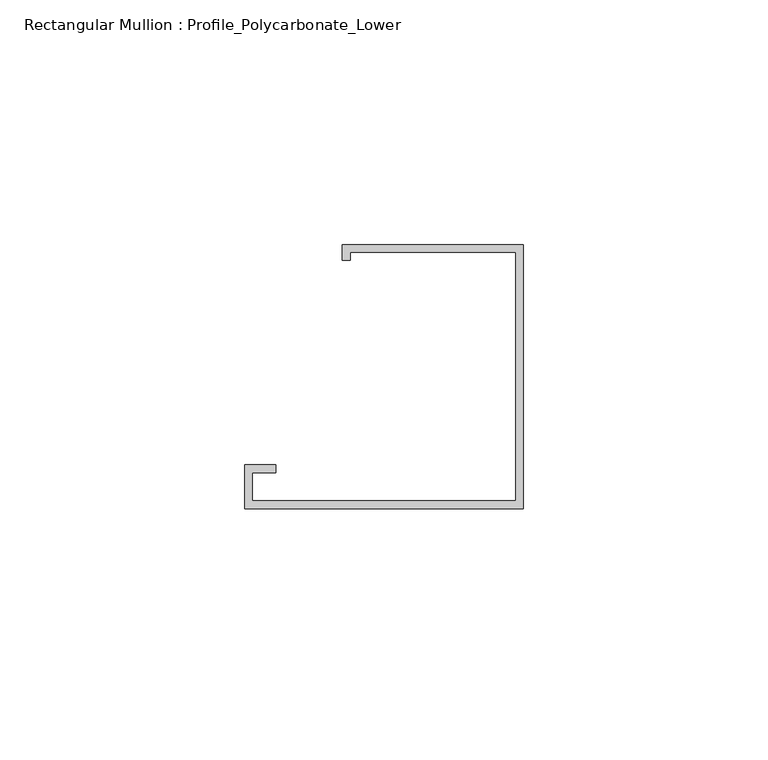
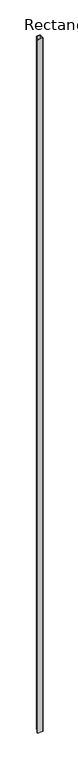
"""IFC4 building model written with IfcOpenShell, lengths in millimetres: member geometry, Rectangular Mullion : Profile_Polycarbonate_Lower."""

from ifc_helpers import new_model, si_unit, frame, origin, place, context, project, spatial, polyline, outline, extrude, source, transform, mapped, element, save


def rectangular_mullion_profile_polycarbonate_lower_ec7f4152(model_context):
    return source(origin(), model_context, "Body", "SweptSolid", [
        extrude(outline(polyline([(0.0, -28.984575), (-56.9976, -28.984575), (-56.9976, -19.992975), (-50.6476, -19.992975), (-50.6476, -21.580475), (-55.4101, -21.580475), (-55.4101, -27.397075), (-1.5875, -27.397075), (-1.5875, 23.428325), (-35.3949, 23.428325), (-35.3949, 21.840825), (-36.9824, 21.840825), (-36.9824, 25.015825), (0.0, 25.015825), (0.0, -28.984575)])), frame((0.0, 0.0, -7626.8283931), z_axis=(0.0, 0.0, 1.0), x_axis=(1.0, 0.0, 0.0)), (0.0, 0.0, 1.0), 7626.8283931),
    ])


if __name__ == "__main__":
    model = new_model("IFC4")
    model_context = context("Model", 3, world=origin())
    ifc_project = project(units=[si_unit("LENGTHUNIT", "METRE", prefix="MILLI")], contexts=[model_context])
    site = spatial("IfcSite", under=ifc_project)
    building = spatial("IfcBuilding", under=site)
    placement = place(None, origin())
    rectangular_mullion_profile_polycarbonate_lower_shape = rectangular_mullion_profile_polycarbonate_lower_ec7f4152(model_context)
    element("IfcMember", 1, ObjectType="Rectangular Mullion : Profile_Polycarbonate_Lower", at=placement, inside=building, context=model_context, shape_type="MappedRepresentation", body=[
        mapped(rectangular_mullion_profile_polycarbonate_lower_shape, transform((0.0, 0.0, 0.0), x_axis=(1.0, 0.0, 0.0), y_axis=(0.0, 1.0, 0.0), z_axis=(0.0, 0.0, 1.0))),
    ])
    save(model, "model.ifc")

# Revit data of these elements
# Type "Rectangular Mullion : Profile_Polycarbonate_Lower"
#   built-in parameter 1007322 = 0.177167 (stored number, unit not read)
#   built-in parameter 1007321 = 0 (stored number, unit not read)
#   built-in parameter 1007320 = 0.00520833 (stored number, unit not read)
